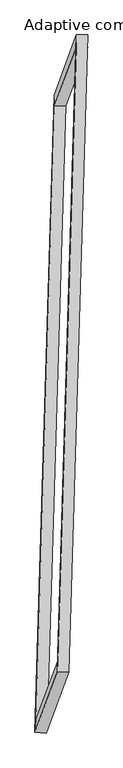
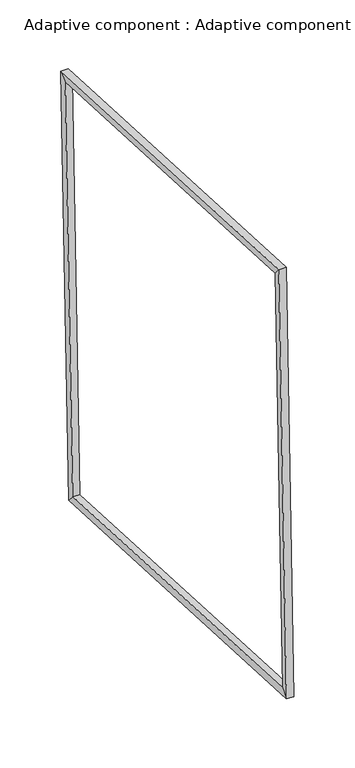
"""IFC4 building model written with IfcOpenShell, lengths in millimetres: proxy geometry, Adaptive component : Adaptive component."""

from ifc_helpers import new_model, si_unit, origin, place, context, project, spatial, faceted_brep, source, transform, mapped, element, save


def adaptive_component_adaptive_component_82e2782b(model_context):
    return source(origin(), model_context, "Body", "Brep", [
        faceted_brep([(95.9758804, 1559.0322514, 3118.0613771), (161.0007761, 1558.8810059, 3117.7774167), (33.999322, 1215.5614832, -753.4333898), (-30.9061833, 1216.0354733, -749.5102184), (93.728255, 1488.5501759, 3059.1217077), (-28.9095631, 1157.0267495, -679.0783829), (158.7531507, 1488.3989304, 3058.8377472), (35.9959423, 1156.5527594, -683.0015542), (-75.1226675, -2401.5915536, -429.0651318), (-139.918386, -2397.4783713, -425.468305), (-134.0189163, -2327.1162538, -366.6378018), (-69.2231978, -2331.2294361, -370.2346286), (51.8787866, -2058.2720309, 3442.1456746), (-13.0363223, -2054.4815932, 3442.1032905), (-11.3810982, -1995.5928274, 3371.5622887), (53.5340107, -1999.3832652, 3371.6046729)], [[[0, 1, 2, 3]], [[4, 0, 3, 5]], [[6, 4, 5, 7]], [[1, 6, 7, 2]], [[3, 2, 8, 9]], [[5, 3, 9, 10]], [[7, 5, 10, 11]], [[2, 7, 11, 8]], [[9, 8, 12, 13]], [[10, 9, 13, 14]], [[11, 10, 14, 15]], [[8, 11, 15, 12]], [[13, 12, 1, 0]], [[14, 13, 0, 4]], [[15, 14, 4, 6]], [[12, 15, 6, 1]]]),
    ])


if __name__ == "__main__":
    model = new_model("IFC4")
    model_context = context("Model", 3, world=origin())
    ifc_project = project(units=[si_unit("LENGTHUNIT", "METRE", prefix="MILLI")], contexts=[model_context])
    site = spatial("IfcSite", under=ifc_project)
    building = spatial("IfcBuilding", under=site)
    placement = place(None, origin())
    adaptive_component_adaptive_component_shape = adaptive_component_adaptive_component_82e2782b(model_context)
    element("IfcBuildingElementProxy", 1, Name="Adaptive component : Adaptive component", ObjectType="Adaptive component : Adaptive component", at=placement, inside=building, context=model_context, shape_type="MappedRepresentation", body=[
        mapped(adaptive_component_adaptive_component_shape, transform((0.0, 0.0, 0.0), x_axis=(1.0, 0.0, 0.0), y_axis=(0.0, 1.0, 0.0), z_axis=(0.0, 0.0, 1.0))),
    ])
    save(model, "model.ifc")

# Revit data of these elements
# Type "Adaptive component : Adaptive component"
#   r [instance default] = 2063.125 mm
#   2r [instance default] = 4126.251 mm
#   Number [instance default] = 5
#   Default Elevation = 0
# Element 1 (IfcBuildingElementProxy, "Adaptive component : Adaptive component")
#   r = 2566.677 mm
#   2r = 5133.354 mm
#   Number = 23
